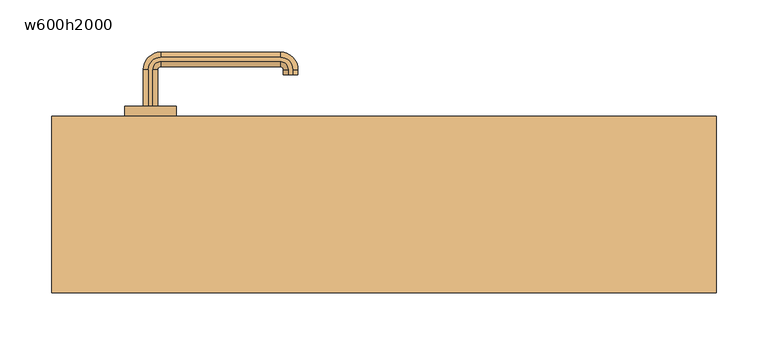
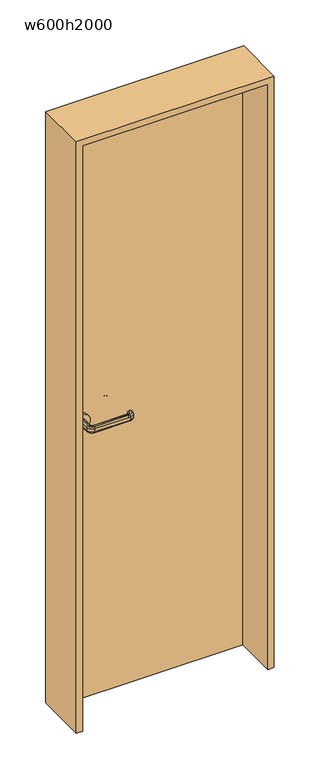
"""IFC4 building model written with IfcOpenShell, lengths in millimetres: door geometry, 片開き : w600h2000."""

from ifc_helpers import new_model, si_unit, point, frame, frame_2d, origin, origin_with_axes, place, context, project, spatial, polyline, circle_curve, ellipse_curve, trimmed, segment, composite_curve, outline, extrude, source, transform, mapped, element, save
from ifc_brep_helpers import plane_surface, cylinder_surface, revolved_surface, advanced_brep


def w600h2000_ea82102f(model_context):
    return source(origin(), model_context, "Body", "SolidModel", [
        advanced_brep(
        [(-227.0, 95.0, 960.0), (-232.0, 95.0, 955.0), (-232.0, 95.0, 945.0477623), (-227.0, 95.0, 940.0477623), (-223.0, 95.0, 940.0477623), (-218.0, 95.0, 945.0477623), (-218.0, 95.0, 955.0), (-223.0, 95.0, 960.0), (-227.0, 130.0, 960.0), (-232.0, 130.0, 955.0), (-232.0, 130.0, 945.0477623), (-227.0, 130.0, 940.0477623), (-215.0, 142.0, 940.0477623), (-100.0, 142.0, 940.0477623), (-88.0, 130.0, 940.0477623), (-88.0, 125.0, 940.0477623), (-92.0, 125.0, 940.0477623), (-92.0, 130.0, 940.0477623), (-100.0, 138.0, 940.0477623), (-215.0, 138.0, 940.0477623), (-223.0, 130.0, 940.0477623), (-218.0, 130.0, 945.0477623), (-218.0, 130.0, 955.0), (-223.0, 130.0, 960.0), (-215.0, 138.0, 960.0), (-100.0, 138.0, 960.0), (-92.0, 130.0, 960.0), (-92.0, 125.0, 960.0), (-88.0, 125.0, 960.0), (-88.0, 130.0, 960.0), (-100.0, 142.0, 960.0), (-215.0, 142.0, 960.0), (-215.0, 147.0, 955.0), (-215.0, 147.0, 945.0477623), (-215.0, 133.0, 945.0477623), (-215.0, 133.0, 955.0), (-100.0, 147.0, 955.0), (-100.0, 147.0, 945.0477623), (-100.0, 133.0, 945.0477623), (-100.0, 133.0, 955.0), (-83.0, 130.0, 955.0), (-83.0, 130.0, 945.0477623), (-97.0, 130.0, 945.0477623), (-97.0, 130.0, 955.0), (-97.0, 125.0, 955.0), (-97.0, 125.0, 945.0477623), (-83.0, 125.0, 945.0477623), (-83.0, 125.0, 955.0)],
        [
            (0, 1, circle_curve(frame((-227.0, 95.0, 955.0), z_axis=(0.0, -1.0, 0.0), x_axis=(-1.0, 0.0, 0.0)), 5.0)),
            (1, 2),
            (2, 3, circle_curve(frame((-227.0, 95.0, 945.0477623), z_axis=(0.0, -1.0, 0.0), x_axis=(-1.0, 0.0, 0.0)), 5.0)),
            (3, 4),
            (4, 5, circle_curve(frame((-223.0, 95.0, 945.0477623), z_axis=(0.0, -1.0, 0.0), x_axis=(-1.0, 0.0, 0.0)), 5.0)),
            (5, 6),
            (6, 7, circle_curve(frame((-223.0, 95.0, 955.0), z_axis=(0.0, -1.0, 0.0), x_axis=(-1.0, 0.0, 0.0)), 5.0)),
            (7, 0),
            (0, 8),
            (8, 9, circle_curve(frame((-227.0, 130.0, 955.0), z_axis=(0.0, -1.0, 0.0), x_axis=(-1.0, 0.0, 0.0)), 5.0)),
            (9, 1),
            (9, 10),
            (10, 2),
            (10, 11, circle_curve(frame((-227.0, 130.0, 945.0477623), z_axis=(0.0, -1.0, 0.0), x_axis=(-1.0, 0.0, 0.0)), 5.0)),
            (11, 3),
            (11, 12, circle_curve(frame((-215.0, 130.0, 940.0477623), z_axis=(0.0, 0.0, -1.0), x_axis=(-1.0, 0.0, 0.0)), 12.0)),
            (12, 13),
            (13, 14, circle_curve(frame((-100.0, 130.0, 940.0477623), z_axis=(0.0, 0.0, -1.0), x_axis=(0.0, 1.0, 0.0)), 12.0)),
            (14, 15),
            (15, 16),
            (16, 17),
            (17, 18, circle_curve(frame((-100.0, 130.0, 940.0477623), z_axis=(0.0, 0.0, 1.0), x_axis=(0.0, 1.0, 0.0)), 8.0)),
            (18, 19),
            (19, 20, circle_curve(frame((-215.0, 130.0, 940.0477623), z_axis=(0.0, 0.0, 1.0), x_axis=(-1.0, 0.0, 0.0)), 8.0)),
            (20, 4),
            (20, 21, circle_curve(frame((-223.0, 130.0, 945.0477623), z_axis=(0.0, -1.0, 0.0), x_axis=(-1.0, 0.0, 0.0)), 5.0)),
            (21, 5),
            (21, 22),
            (22, 6),
            (22, 23, circle_curve(frame((-223.0, 130.0, 955.0), z_axis=(0.0, -1.0, 0.0), x_axis=(-1.0, 0.0, 0.0)), 5.0)),
            (23, 7),
            (23, 24, circle_curve(frame((-215.0, 130.0, 960.0), z_axis=(0.0, 0.0, -1.0), x_axis=(-1.0, 0.0, 0.0)), 8.0)),
            (24, 25),
            (25, 26, circle_curve(frame((-100.0, 130.0, 960.0), z_axis=(0.0, 0.0, -1.0), x_axis=(0.0, 1.0, 0.0)), 8.0)),
            (26, 27),
            (27, 28),
            (28, 29),
            (29, 30, circle_curve(frame((-100.0, 130.0, 960.0), z_axis=(0.0, 0.0, 1.0), x_axis=(0.0, 1.0, 0.0)), 12.0)),
            (30, 31),
            (31, 8, circle_curve(frame((-215.0, 130.0, 960.0), z_axis=(0.0, 0.0, 1.0), x_axis=(-1.0, 0.0, 0.0)), 12.0)),
            (32, 9, circle_curve(frame((-215.0, 130.0, 955.0), z_axis=(0.0, 0.0, 1.0), x_axis=(-1.0, 0.0, 0.0)), 17.0)),
            (31, 32, circle_curve(frame((-215.0, 142.0, 955.0), z_axis=(-1.0, 0.0, 0.0), x_axis=(0.0, 1.0, 0.0)), 5.0)),
            (33, 10, circle_curve(frame((-215.0, 130.0, 945.0477623), z_axis=(0.0, 0.0, 1.0), x_axis=(-1.0, 0.0, 0.0)), 17.0)),
            (32, 33),
            (33, 12, circle_curve(frame((-215.0, 142.0, 945.0477623), z_axis=(-1.0, 0.0, 0.0), x_axis=(0.0, 1.0, 0.0)), 5.0)),
            (34, 21, circle_curve(frame((-215.0, 130.0, 945.0477623), z_axis=(0.0, 0.0, 1.0), x_axis=(-1.0, 0.0, 0.0)), 3.0)),
            (19, 34, circle_curve(frame((-215.0, 138.0, 945.0477623), z_axis=(-1.0, 0.0, 0.0), x_axis=(0.0, 1.0, 0.0)), 5.0)),
            (35, 22, circle_curve(frame((-215.0, 130.0, 955.0), z_axis=(0.0, 0.0, 1.0), x_axis=(-1.0, 0.0, 0.0)), 3.0)),
            (34, 35),
            (35, 24, circle_curve(frame((-215.0, 138.0, 955.0), z_axis=(-1.0, 0.0, 0.0), x_axis=(0.0, 1.0, 0.0)), 5.0)),
            (30, 36, circle_curve(frame((-100.0, 142.0, 955.0), z_axis=(-1.0, 0.0, 0.0), x_axis=(0.0, 1.0, 0.0)), 5.0)),
            (36, 32),
            (36, 37),
            (37, 33),
            (37, 13, circle_curve(frame((-100.0, 142.0, 945.0477623), z_axis=(-1.0, 0.0, 0.0), x_axis=(0.0, 1.0, 0.0)), 5.0)),
            (18, 38, circle_curve(frame((-100.0, 138.0, 945.0477623), z_axis=(-1.0, 0.0, 0.0), x_axis=(0.0, 1.0, 0.0)), 5.0)),
            (38, 34),
            (38, 39),
            (39, 35),
            (39, 25, circle_curve(frame((-100.0, 138.0, 955.0), z_axis=(-1.0, 0.0, 0.0), x_axis=(0.0, 1.0, 0.0)), 5.0)),
            (40, 36, circle_curve(frame((-100.0, 130.0, 955.0), z_axis=(0.0, 0.0, 1.0), x_axis=(0.0, 1.0, 0.0)), 17.0)),
            (29, 40, circle_curve(frame((-88.0, 130.0, 955.0), z_axis=(0.0, 1.0, 0.0), x_axis=(1.0, 0.0, 0.0)), 5.0)),
            (41, 37, circle_curve(frame((-100.0, 130.0, 945.0477623), z_axis=(0.0, 0.0, 1.0), x_axis=(0.0, 1.0, 0.0)), 17.0)),
            (40, 41),
            (41, 14, circle_curve(frame((-88.0, 130.0, 945.0477623), z_axis=(0.0, 1.0, 0.0), x_axis=(1.0, 0.0, 0.0)), 5.0)),
            (42, 38, circle_curve(frame((-100.0, 130.0, 945.0477623), z_axis=(0.0, 0.0, 1.0), x_axis=(0.0, 1.0, 0.0)), 3.0)),
            (17, 42, circle_curve(frame((-92.0, 130.0, 945.0477623), z_axis=(0.0, 1.0, 0.0), x_axis=(1.0, 0.0, 0.0)), 5.0)),
            (43, 39, circle_curve(frame((-100.0, 130.0, 955.0), z_axis=(0.0, 0.0, 1.0), x_axis=(0.0, 1.0, 0.0)), 3.0)),
            (42, 43),
            (43, 26, circle_curve(frame((-92.0, 130.0, 955.0), z_axis=(0.0, 1.0, 0.0), x_axis=(1.0, 0.0, 0.0)), 5.0)),
            (27, 44, circle_curve(frame((-92.0, 125.0, 955.0), z_axis=(0.0, -1.0, 0.0), x_axis=(1.0, 0.0, 0.0)), 5.0)),
            (44, 45),
            (45, 16, circle_curve(frame((-92.0, 125.0, 945.0477623), z_axis=(0.0, -1.0, 0.0), x_axis=(1.0, 0.0, 0.0)), 5.0)),
            (15, 46, circle_curve(frame((-88.0, 125.0, 945.0477623), z_axis=(0.0, -1.0, 0.0), x_axis=(1.0, 0.0, 0.0)), 5.0)),
            (46, 47),
            (47, 28, circle_curve(frame((-88.0, 125.0, 955.0), z_axis=(0.0, -1.0, 0.0), x_axis=(1.0, 0.0, 0.0)), 5.0)),
            (47, 40),
            (46, 41),
            (45, 42),
            (44, 43),
        ],
        [
            plane_surface(frame((-235.198039, 95.0, 950.0), z_axis=(0.0, -1.0, 0.0), x_axis=(0.0, 0.0, 1.0))),
            cylinder_surface(frame((-227.0, 95.0, 955.0), z_axis=(0.0, -1.0, 0.0), x_axis=(-1.0, 0.0, 0.0)), 5.0),
            plane_surface(frame((-232.0, 95.0, 955.0), z_axis=(-1.0, 0.0, 0.0), x_axis=(0.0, 1.0, 0.0))),
            cylinder_surface(frame((-227.0, 95.0, 945.0477623), z_axis=(0.0, -1.0, 0.0), x_axis=(-1.0, 0.0, 0.0)), 5.0),
            plane_surface(frame((-227.0, 95.0, 940.0477623), z_axis=(0.0, 0.0, -1.0), x_axis=(0.0, 1.0, 0.0))),
            cylinder_surface(frame((-223.0, 95.0, 945.0477623), z_axis=(0.0, -1.0, 0.0), x_axis=(-1.0, 0.0, 0.0)), 5.0),
            plane_surface(frame((-218.0, 95.0, 945.0477623), z_axis=(1.0, 0.0, 0.0), x_axis=(0.0, 1.0, 0.0))),
            cylinder_surface(frame((-223.0, 95.0, 955.0), z_axis=(0.0, -1.0, 0.0), x_axis=(-1.0, 0.0, 0.0)), 5.0),
            plane_surface(frame((-223.0, 95.0, 960.0), z_axis=(0.0, 0.0, 1.0), x_axis=(0.0, 1.0, 0.0))),
            revolved_surface(trimmed(ellipse_curve(frame((-227.0, 130.0, 955.0), z_axis=(0.0, -1.0, 0.0), x_axis=(-1.0, 0.0, 0.0)), 5.0, 5.0), [point((-227.0, 130.0, 960.0))], [point((-232.0, 130.0, 955.0))], True, "CARTESIAN"), (-215.0, 130.0, 950.0), (0.0, 0.0, -1.0)),
            cylinder_surface(frame((-215.0, 130.0, 950.0), z_axis=(0.0, 0.0, -1.0), x_axis=(-1.0, 0.0, 0.0)), 17.0),
            revolved_surface(trimmed(ellipse_curve(frame((-227.0, 130.0, 945.0477623), z_axis=(0.0, -1.0, 0.0), x_axis=(-1.0, 0.0, 0.0)), 5.0, 5.0), [point((-232.0, 130.0, 945.0477623))], [point((-227.0, 130.0, 940.0477623))], True, "CARTESIAN"), (-215.0, 130.0, 950.0), (0.0, 0.0, -1.0)),
            revolved_surface(trimmed(ellipse_curve(frame((-223.0, 130.0, 945.0477623), z_axis=(0.0, -1.0, 0.0), x_axis=(-1.0, 0.0, 0.0)), 5.0, 5.0), [point((-223.0, 130.0, 940.0477623))], [point((-218.0, 130.0, 945.0477623))], True, "CARTESIAN"), (-215.0, 130.0, 950.0), (0.0, 0.0, -1.0)),
            revolved_surface(polyline([(-218.0, 130.0, 945.0477623), (-218.0, 130.0, 955.0)]), (-215.0, 130.0, 950.0), (0.0, 0.0, -1.0)),
            revolved_surface(trimmed(ellipse_curve(frame((-223.0, 130.0, 955.0), z_axis=(0.0, -1.0, 0.0), x_axis=(-1.0, 0.0, 0.0)), 5.0, 5.0), [point((-218.0, 130.0, 955.0))], [point((-223.0, 130.0, 960.0))], True, "CARTESIAN"), (-215.0, 130.0, 950.0), (0.0, 0.0, -1.0)),
            cylinder_surface(frame((-215.0, 142.0, 955.0), z_axis=(-1.0, 0.0, 0.0), x_axis=(0.0, 1.0, 0.0)), 5.0),
            plane_surface(frame((-215.0, 147.0, 955.0), z_axis=(0.0, 1.0, 0.0), x_axis=(1.0, 0.0, 0.0))),
            cylinder_surface(frame((-215.0, 142.0, 945.0477623), z_axis=(-1.0, 0.0, 0.0), x_axis=(0.0, 1.0, 0.0)), 5.0),
            cylinder_surface(frame((-215.0, 138.0, 945.0477623), z_axis=(-1.0, 0.0, 0.0), x_axis=(0.0, 1.0, 0.0)), 5.0),
            plane_surface(frame((-215.0, 133.0, 945.0477623), z_axis=(0.0, -1.0, 0.0), x_axis=(1.0, 0.0, 0.0))),
            cylinder_surface(frame((-215.0, 138.0, 955.0), z_axis=(-1.0, 0.0, 0.0), x_axis=(0.0, 1.0, 0.0)), 5.0),
            revolved_surface(trimmed(ellipse_curve(frame((-100.0, 142.0, 955.0), z_axis=(-1.0, 0.0, 0.0), x_axis=(0.0, 1.0, 0.0)), 5.0, 5.0), [point((-100.0, 142.0, 960.0))], [point((-100.0, 147.0, 955.0))], True, "CARTESIAN"), (-100.0, 130.0, 950.0), (0.0, 0.0, -1.0)),
            cylinder_surface(frame((-100.0, 130.0, 950.0), z_axis=(0.0, 0.0, -1.0), x_axis=(0.0, 1.0, 0.0)), 17.0),
            revolved_surface(trimmed(ellipse_curve(frame((-100.0, 142.0, 945.0477623), z_axis=(-1.0, 0.0, 0.0), x_axis=(0.0, 1.0, 0.0)), 5.0, 5.0), [point((-100.0, 147.0, 945.0477623))], [point((-100.0, 142.0, 940.0477623))], True, "CARTESIAN"), (-100.0, 130.0, 950.0), (0.0, 0.0, -1.0)),
            revolved_surface(trimmed(ellipse_curve(frame((-100.0, 138.0, 945.0477623), z_axis=(-1.0, 0.0, 0.0), x_axis=(0.0, 1.0, 0.0)), 5.0, 5.0), [point((-100.0, 138.0, 940.0477623))], [point((-100.0, 133.0, 945.0477623))], True, "CARTESIAN"), (-100.0, 130.0, 950.0), (0.0, 0.0, -1.0)),
            revolved_surface(polyline([(-100.0, 133.0, 945.0477623), (-100.0, 133.0, 955.0)]), (-100.0, 130.0, 950.0), (0.0, 0.0, -1.0)),
            revolved_surface(trimmed(ellipse_curve(frame((-100.0, 138.0, 955.0), z_axis=(-1.0, 0.0, 0.0), x_axis=(0.0, 1.0, 0.0)), 5.0, 5.0), [point((-100.0, 133.0, 955.0))], [point((-100.0, 138.0, 960.0))], True, "CARTESIAN"), (-100.0, 130.0, 950.0), (0.0, 0.0, -1.0)),
            plane_surface(frame((-100.198039, 125.0, 950.0), z_axis=(0.0, -1.0, 0.0), x_axis=(0.0, 0.0, -1.0))),
            cylinder_surface(frame((-88.0, 130.0, 955.0), z_axis=(0.0, 1.0, 0.0), x_axis=(1.0, 0.0, 0.0)), 5.0),
            plane_surface(frame((-83.0, 130.0, 955.0), z_axis=(1.0, 0.0, 0.0), x_axis=(0.0, -1.0, 0.0))),
            cylinder_surface(frame((-88.0, 130.0, 945.0477623), z_axis=(0.0, 1.0, 0.0), x_axis=(1.0, 0.0, 0.0)), 5.0),
            cylinder_surface(frame((-92.0, 130.0, 945.0477623), z_axis=(0.0, 1.0, 0.0), x_axis=(1.0, 0.0, 0.0)), 5.0),
            plane_surface(frame((-97.0, 130.0, 945.0477623), z_axis=(-1.0, 0.0, 0.0), x_axis=(0.0, -1.0, 0.0))),
            cylinder_surface(frame((-92.0, 130.0, 955.0), z_axis=(0.0, 1.0, 0.0), x_axis=(1.0, 0.0, 0.0)), 5.0),
        ],
        [
            (0, [[1, 2, 3, 4, 5, 6, 7, 8]]),
            (1, [[-1, 9, 10, 11]]),
            (2, [[-2, -11, 12, 13]]),
            (3, [[-3, -13, 14, 15]]),
            (4, [[-4, -15, 16, 17, 18, 19, 20, 21, 22, 23, 24, 25]]),
            (5, [[-5, -25, 26, 27]]),
            (6, [[-6, -27, 28, 29]]),
            (7, [[-7, -29, 30, 31]]),
            (8, [[-8, -31, 32, 33, 34, 35, 36, 37, 38, 39, 40, -9]]),
            (9, [[41, -10, -40, 42]]),
            (10, [[43, -12, -41, 44]]),
            (11, [[-16, -14, -43, 45]]),
            (12, [[46, -26, -24, 47]]),
            (13, [[48, -28, -46, 49]]),
            (14, [[-32, -30, -48, 50]]),
            (15, [[-42, -39, 51, 52]]),
            (16, [[-44, -52, 53, 54]]),
            (17, [[-45, -54, 55, -17]]),
            (18, [[-47, -23, 56, 57]]),
            (19, [[-49, -57, 58, 59]]),
            (20, [[-50, -59, 60, -33]]),
            (21, [[61, -51, -38, 62]]),
            (22, [[63, -53, -61, 64]]),
            (23, [[-18, -55, -63, 65]]),
            (24, [[66, -56, -22, 67]]),
            (25, [[68, -58, -66, 69]]),
            (26, [[-34, -60, -68, 70]]),
            (27, [[-36, 71, 72, 73, -20, 74, 75, 76]]),
            (28, [[-62, -37, -76, 77]]),
            (29, [[-64, -77, -75, 78]]),
            (30, [[-65, -78, -74, -19]]),
            (31, [[-67, -21, -73, 79]]),
            (32, [[-69, -79, -72, 80]]),
            (33, [[-70, -80, -71, -35]]),
        ],
    ),
        advanced_brep(
        [(-223.0, 45.0, 940.0), (-227.0, 45.0, 940.0), (-232.0, 45.0, 945.0), (-232.0, 45.0, 955.0), (-227.0, 45.0, 960.0), (-223.0, 45.0, 960.0), (-218.0, 45.0, 955.0), (-218.0, 45.0, 945.0), (-223.0, 10.0, 940.0), (-215.0, 2.0, 940.0), (-100.0, 2.0, 940.0), (-92.0, 10.0, 940.0), (-92.0, 15.0, 940.0), (-88.0, 15.0, 940.0), (-88.0, 10.0, 940.0), (-100.0, -2.0, 940.0), (-215.0, -2.0, 940.0), (-227.0, 10.0, 940.0), (-232.0, 10.0, 945.0), (-232.0, 10.0, 955.0), (-227.0, 10.0, 960.0), (-215.0, -2.0, 960.0), (-100.0, -2.0, 960.0), (-88.0, 10.0, 960.0), (-88.0, 15.0, 960.0), (-92.0, 15.0, 960.0), (-92.0, 10.0, 960.0), (-100.0, 2.0, 960.0), (-215.0, 2.0, 960.0), (-223.0, 10.0, 960.0), (-218.0, 10.0, 955.0), (-218.0, 10.0, 945.0), (-215.0, -7.0, 945.0), (-215.0, -7.0, 955.0), (-215.0, 7.0, 955.0), (-215.0, 7.0, 945.0), (-100.0, -7.0, 945.0), (-100.0, -7.0, 955.0), (-100.0, 7.0, 955.0), (-100.0, 7.0, 945.0), (-83.0, 10.0, 945.0), (-83.0, 10.0, 955.0), (-97.0, 10.0, 955.0), (-97.0, 10.0, 945.0), (-97.0, 15.0, 945.0), (-97.0, 15.0, 955.0), (-83.0, 15.0, 955.0), (-83.0, 15.0, 945.0)],
        [
            (0, 1),
            (1, 2, circle_curve(frame((-227.0, 45.0, 945.0), z_axis=(0.0, 1.0, 0.0), x_axis=(1.0, 0.0, 0.0)), 5.0)),
            (2, 3),
            (3, 4, circle_curve(frame((-227.0, 45.0, 955.0), z_axis=(0.0, 1.0, 0.0), x_axis=(1.0, 0.0, 0.0)), 5.0)),
            (4, 5),
            (5, 6, circle_curve(frame((-223.0, 45.0, 955.0), z_axis=(0.0, 1.0, 0.0), x_axis=(1.0, 0.0, 0.0)), 5.0)),
            (6, 7),
            (7, 0, circle_curve(frame((-223.0, 45.0, 945.0), z_axis=(0.0, 1.0, 0.0), x_axis=(1.0, 0.0, 0.0)), 5.0)),
            (0, 8),
            (8, 9, circle_curve(frame((-215.0, 10.0, 940.0), z_axis=(0.0, 0.0, 1.0), x_axis=(-1.0, 0.0, 0.0)), 8.0)),
            (9, 10),
            (10, 11, circle_curve(frame((-100.0, 10.0, 940.0), z_axis=(0.0, 0.0, 1.0), x_axis=(0.0, -1.0, 0.0)), 8.0)),
            (11, 12),
            (12, 13),
            (13, 14),
            (14, 15, circle_curve(frame((-100.0, 10.0, 940.0), z_axis=(0.0, 0.0, -1.0), x_axis=(0.0, -1.0, 0.0)), 12.0)),
            (15, 16),
            (16, 17, circle_curve(frame((-215.0, 10.0, 940.0), z_axis=(0.0, 0.0, -1.0), x_axis=(-1.0, 0.0, 0.0)), 12.0)),
            (17, 1),
            (17, 18, circle_curve(frame((-227.0, 10.0, 945.0), z_axis=(0.0, 1.0, 0.0), x_axis=(1.0, 0.0, 0.0)), 5.0)),
            (18, 2),
            (18, 19),
            (19, 3),
            (19, 20, circle_curve(frame((-227.0, 10.0, 955.0), z_axis=(0.0, 1.0, 0.0), x_axis=(1.0, 0.0, 0.0)), 5.0)),
            (20, 4),
            (20, 21, circle_curve(frame((-215.0, 10.0, 960.0), z_axis=(0.0, 0.0, 1.0), x_axis=(-1.0, 0.0, 0.0)), 12.0)),
            (21, 22),
            (22, 23, circle_curve(frame((-100.0, 10.0, 960.0), z_axis=(0.0, 0.0, 1.0), x_axis=(0.0, -1.0, 0.0)), 12.0)),
            (23, 24),
            (24, 25),
            (25, 26),
            (26, 27, circle_curve(frame((-100.0, 10.0, 960.0), z_axis=(0.0, 0.0, -1.0), x_axis=(0.0, -1.0, 0.0)), 8.0)),
            (27, 28),
            (28, 29, circle_curve(frame((-215.0, 10.0, 960.0), z_axis=(0.0, 0.0, -1.0), x_axis=(-1.0, 0.0, 0.0)), 8.0)),
            (29, 5),
            (29, 30, circle_curve(frame((-223.0, 10.0, 955.0), z_axis=(0.0, 1.0, 0.0), x_axis=(1.0, 0.0, 0.0)), 5.0)),
            (30, 6),
            (30, 31),
            (31, 7),
            (31, 8, circle_curve(frame((-223.0, 10.0, 945.0), z_axis=(0.0, 1.0, 0.0), x_axis=(1.0, 0.0, 0.0)), 5.0)),
            (32, 18, circle_curve(frame((-215.0, 10.0, 945.0), z_axis=(0.0, 0.0, -1.0), x_axis=(-1.0, 0.0, 0.0)), 17.0)),
            (16, 32, circle_curve(frame((-215.0, -2.0, 945.0), z_axis=(-1.0, 0.0, 0.0), x_axis=(0.0, 1.0, 0.0)), 5.0)),
            (33, 19, circle_curve(frame((-215.0, 10.0, 955.0), z_axis=(0.0, 0.0, -1.0), x_axis=(-1.0, 0.0, 0.0)), 17.0)),
            (32, 33),
            (33, 21, circle_curve(frame((-215.0, -2.0, 955.0), z_axis=(-1.0, 0.0, 0.0), x_axis=(0.0, 1.0, 0.0)), 5.0)),
            (34, 30, circle_curve(frame((-215.0, 10.0, 955.0), z_axis=(0.0, 0.0, -1.0), x_axis=(-1.0, 0.0, 0.0)), 3.0)),
            (28, 34, circle_curve(frame((-215.0, 2.0, 955.0), z_axis=(-1.0, 0.0, 0.0), x_axis=(0.0, 1.0, 0.0)), 5.0)),
            (35, 31, circle_curve(frame((-215.0, 10.0, 945.0), z_axis=(0.0, 0.0, -1.0), x_axis=(-1.0, 0.0, 0.0)), 3.0)),
            (34, 35),
            (35, 9, circle_curve(frame((-215.0, 2.0, 945.0), z_axis=(-1.0, 0.0, 0.0), x_axis=(0.0, 1.0, 0.0)), 5.0)),
            (15, 36, circle_curve(frame((-100.0, -2.0, 945.0), z_axis=(-1.0, 0.0, 0.0), x_axis=(0.0, 1.0, 0.0)), 5.0)),
            (36, 32),
            (36, 37),
            (37, 33),
            (37, 22, circle_curve(frame((-100.0, -2.0, 955.0), z_axis=(-1.0, 0.0, 0.0), x_axis=(0.0, 1.0, 0.0)), 5.0)),
            (27, 38, circle_curve(frame((-100.0, 2.0, 955.0), z_axis=(-1.0, 0.0, 0.0), x_axis=(0.0, 1.0, 0.0)), 5.0)),
            (38, 34),
            (38, 39),
            (39, 35),
            (39, 10, circle_curve(frame((-100.0, 2.0, 945.0), z_axis=(-1.0, 0.0, 0.0), x_axis=(0.0, 1.0, 0.0)), 5.0)),
            (40, 36, circle_curve(frame((-100.0, 10.0, 945.0), z_axis=(0.0, 0.0, -1.0), x_axis=(0.0, -1.0, 0.0)), 17.0)),
            (14, 40, circle_curve(frame((-88.0, 10.0, 945.0), z_axis=(0.0, -1.0, 0.0), x_axis=(-1.0, 0.0, 0.0)), 5.0)),
            (41, 37, circle_curve(frame((-100.0, 10.0, 955.0), z_axis=(0.0, 0.0, -1.0), x_axis=(0.0, -1.0, 0.0)), 17.0)),
            (40, 41),
            (41, 23, circle_curve(frame((-88.0, 10.0, 955.0), z_axis=(0.0, -1.0, 0.0), x_axis=(-1.0, 0.0, 0.0)), 5.0)),
            (42, 38, circle_curve(frame((-100.0, 10.0, 955.0), z_axis=(0.0, 0.0, -1.0), x_axis=(0.0, -1.0, 0.0)), 3.0)),
            (26, 42, circle_curve(frame((-92.0, 10.0, 955.0), z_axis=(0.0, -1.0, 0.0), x_axis=(-1.0, 0.0, 0.0)), 5.0)),
            (43, 39, circle_curve(frame((-100.0, 10.0, 945.0), z_axis=(0.0, 0.0, -1.0), x_axis=(0.0, -1.0, 0.0)), 3.0)),
            (42, 43),
            (43, 11, circle_curve(frame((-92.0, 10.0, 945.0), z_axis=(0.0, -1.0, 0.0), x_axis=(-1.0, 0.0, 0.0)), 5.0)),
            (12, 44, circle_curve(frame((-92.0, 15.0, 945.0), z_axis=(0.0, 1.0, 0.0), x_axis=(-1.0, 0.0, 0.0)), 5.0)),
            (44, 45),
            (45, 25, circle_curve(frame((-92.0, 15.0, 955.0), z_axis=(0.0, 1.0, 0.0), x_axis=(-1.0, 0.0, 0.0)), 5.0)),
            (24, 46, circle_curve(frame((-88.0, 15.0, 955.0), z_axis=(0.0, 1.0, 0.0), x_axis=(-1.0, 0.0, 0.0)), 5.0)),
            (46, 47),
            (47, 13, circle_curve(frame((-88.0, 15.0, 945.0), z_axis=(0.0, 1.0, 0.0), x_axis=(-1.0, 0.0, 0.0)), 5.0)),
            (47, 40),
            (46, 41),
            (45, 42),
            (44, 43),
        ],
        [
            plane_surface(frame((-235.198039, 45.0, 950.0), z_axis=(0.0, 1.0, 0.0), x_axis=(0.0, 0.0, -1.0))),
            plane_surface(frame((-223.0, 45.0, 940.0), z_axis=(0.0, 0.0, -1.0), x_axis=(0.0, -1.0, 0.0))),
            cylinder_surface(frame((-227.0, 45.0, 945.0), z_axis=(0.0, 1.0, 0.0), x_axis=(1.0, 0.0, 0.0)), 5.0),
            plane_surface(frame((-232.0, 45.0, 945.0), z_axis=(-1.0, 0.0, 0.0), x_axis=(0.0, -1.0, 0.0))),
            cylinder_surface(frame((-227.0, 45.0, 955.0), z_axis=(0.0, 1.0, 0.0), x_axis=(1.0, 0.0, 0.0)), 5.0),
            plane_surface(frame((-227.0, 45.0, 960.0), z_axis=(0.0, 0.0, 1.0), x_axis=(0.0, -1.0, 0.0))),
            cylinder_surface(frame((-223.0, 45.0, 955.0), z_axis=(0.0, 1.0, 0.0), x_axis=(1.0, 0.0, 0.0)), 5.0),
            plane_surface(frame((-218.0, 45.0, 955.0), z_axis=(1.0, 0.0, 0.0), x_axis=(0.0, -1.0, 0.0))),
            cylinder_surface(frame((-223.0, 45.0, 945.0), z_axis=(0.0, 1.0, 0.0), x_axis=(1.0, 0.0, 0.0)), 5.0),
            revolved_surface(trimmed(ellipse_curve(frame((-227.0, 10.0, 945.0), z_axis=(0.0, 1.0, 0.0), x_axis=(1.0, 0.0, 0.0)), 5.0, 5.0), [point((-227.0, 10.0, 940.0))], [point((-232.0, 10.0, 945.0))], True, "CARTESIAN"), (-215.0, 10.0, 950.0), (0.0, 0.0, 1.0)),
            cylinder_surface(frame((-215.0, 10.0, 950.0), z_axis=(0.0, 0.0, 1.0), x_axis=(-1.0, 0.0, 0.0)), 17.0),
            revolved_surface(trimmed(ellipse_curve(frame((-227.0, 10.0, 955.0), z_axis=(0.0, 1.0, 0.0), x_axis=(1.0, 0.0, 0.0)), 5.0, 5.0), [point((-232.0, 10.0, 955.0))], [point((-227.0, 10.0, 960.0))], True, "CARTESIAN"), (-215.0, 10.0, 950.0), (0.0, 0.0, 1.0)),
            revolved_surface(trimmed(ellipse_curve(frame((-223.0, 10.0, 955.0), z_axis=(0.0, 1.0, 0.0), x_axis=(1.0, 0.0, 0.0)), 5.0, 5.0), [point((-223.0, 10.0, 960.0))], [point((-218.0, 10.0, 955.0))], True, "CARTESIAN"), (-215.0, 10.0, 950.0), (0.0, 0.0, 1.0)),
            revolved_surface(polyline([(-218.0, 10.0, 955.0), (-218.0, 10.0, 945.0)]), (-215.0, 10.0, 950.0), (0.0, 0.0, 1.0)),
            revolved_surface(trimmed(ellipse_curve(frame((-223.0, 10.0, 945.0), z_axis=(0.0, 1.0, 0.0), x_axis=(1.0, 0.0, 0.0)), 5.0, 5.0), [point((-218.0, 10.0, 945.0))], [point((-223.0, 10.0, 940.0))], True, "CARTESIAN"), (-215.0, 10.0, 950.0), (0.0, 0.0, 1.0)),
            cylinder_surface(frame((-215.0, -2.0, 945.0), z_axis=(-1.0, 0.0, 0.0), x_axis=(0.0, 1.0, 0.0)), 5.0),
            plane_surface(frame((-215.0, -7.0, 945.0), z_axis=(0.0, -1.0, 0.0), x_axis=(1.0, 0.0, 0.0))),
            cylinder_surface(frame((-215.0, -2.0, 955.0), z_axis=(-1.0, 0.0, 0.0), x_axis=(0.0, 1.0, 0.0)), 5.0),
            cylinder_surface(frame((-215.0, 2.0, 955.0), z_axis=(-1.0, 0.0, 0.0), x_axis=(0.0, 1.0, 0.0)), 5.0),
            plane_surface(frame((-215.0, 7.0, 955.0), z_axis=(0.0, 1.0, 0.0), x_axis=(1.0, 0.0, 0.0))),
            cylinder_surface(frame((-215.0, 2.0, 945.0), z_axis=(-1.0, 0.0, 0.0), x_axis=(0.0, 1.0, 0.0)), 5.0),
            revolved_surface(trimmed(ellipse_curve(frame((-100.0, -2.0, 945.0), z_axis=(-1.0, 0.0, 0.0), x_axis=(0.0, 1.0, 0.0)), 5.0, 5.0), [point((-100.0, -2.0, 940.0))], [point((-100.0, -7.0, 945.0))], True, "CARTESIAN"), (-100.0, 10.0, 950.0), (0.0, 0.0, 1.0)),
            cylinder_surface(frame((-100.0, 10.0, 950.0), z_axis=(0.0, 0.0, 1.0), x_axis=(0.0, -1.0, 0.0)), 17.0),
            revolved_surface(trimmed(ellipse_curve(frame((-100.0, -2.0, 955.0), z_axis=(-1.0, 0.0, 0.0), x_axis=(0.0, 1.0, 0.0)), 5.0, 5.0), [point((-100.0, -7.0, 955.0))], [point((-100.0, -2.0, 960.0))], True, "CARTESIAN"), (-100.0, 10.0, 950.0), (0.0, 0.0, 1.0)),
            revolved_surface(trimmed(ellipse_curve(frame((-100.0, 2.0, 955.0), z_axis=(-1.0, 0.0, 0.0), x_axis=(0.0, 1.0, 0.0)), 5.0, 5.0), [point((-100.0, 2.0, 960.0))], [point((-100.0, 7.0, 955.0))], True, "CARTESIAN"), (-100.0, 10.0, 950.0), (0.0, 0.0, 1.0)),
            revolved_surface(polyline([(-100.0, 7.0, 955.0), (-100.0, 7.0, 945.0)]), (-100.0, 10.0, 950.0), (0.0, 0.0, 1.0)),
            revolved_surface(trimmed(ellipse_curve(frame((-100.0, 2.0, 945.0), z_axis=(-1.0, 0.0, 0.0), x_axis=(0.0, 1.0, 0.0)), 5.0, 5.0), [point((-100.0, 7.0, 945.0))], [point((-100.0, 2.0, 940.0))], True, "CARTESIAN"), (-100.0, 10.0, 950.0), (0.0, 0.0, 1.0)),
            plane_surface(frame((-100.198039, 15.0, 950.0), z_axis=(0.0, 1.0, 0.0), x_axis=(0.0, 0.0, 1.0))),
            cylinder_surface(frame((-88.0, 10.0, 945.0), z_axis=(0.0, -1.0, 0.0), x_axis=(-1.0, 0.0, 0.0)), 5.0),
            plane_surface(frame((-83.0, 10.0, 945.0), z_axis=(1.0, 0.0, 0.0), x_axis=(0.0, 1.0, 0.0))),
            cylinder_surface(frame((-88.0, 10.0, 955.0), z_axis=(0.0, -1.0, 0.0), x_axis=(-1.0, 0.0, 0.0)), 5.0),
            cylinder_surface(frame((-92.0, 10.0, 955.0), z_axis=(0.0, -1.0, 0.0), x_axis=(-1.0, 0.0, 0.0)), 5.0),
            plane_surface(frame((-97.0, 10.0, 955.0), z_axis=(-1.0, 0.0, 0.0), x_axis=(0.0, 1.0, 0.0))),
            cylinder_surface(frame((-92.0, 10.0, 945.0), z_axis=(0.0, -1.0, 0.0), x_axis=(-1.0, 0.0, 0.0)), 5.0),
        ],
        [
            (0, [[1, 2, 3, 4, 5, 6, 7, 8]]),
            (1, [[-1, 9, 10, 11, 12, 13, 14, 15, 16, 17, 18, 19]]),
            (2, [[-2, -19, 20, 21]]),
            (3, [[-3, -21, 22, 23]]),
            (4, [[-4, -23, 24, 25]]),
            (5, [[-5, -25, 26, 27, 28, 29, 30, 31, 32, 33, 34, 35]]),
            (6, [[-6, -35, 36, 37]]),
            (7, [[-7, -37, 38, 39]]),
            (8, [[-8, -39, 40, -9]]),
            (9, [[41, -20, -18, 42]]),
            (10, [[43, -22, -41, 44]]),
            (11, [[-26, -24, -43, 45]]),
            (12, [[46, -36, -34, 47]]),
            (13, [[48, -38, -46, 49]]),
            (14, [[-10, -40, -48, 50]]),
            (15, [[-42, -17, 51, 52]]),
            (16, [[-44, -52, 53, 54]]),
            (17, [[-45, -54, 55, -27]]),
            (18, [[-47, -33, 56, 57]]),
            (19, [[-49, -57, 58, 59]]),
            (20, [[-50, -59, 60, -11]]),
            (21, [[61, -51, -16, 62]]),
            (22, [[63, -53, -61, 64]]),
            (23, [[-28, -55, -63, 65]]),
            (24, [[66, -56, -32, 67]]),
            (25, [[68, -58, -66, 69]]),
            (26, [[-12, -60, -68, 70]]),
            (27, [[71, 72, 73, -30, 74, 75, 76, -14]]),
            (28, [[-62, -15, -76, 77]]),
            (29, [[-64, -77, -75, 78]]),
            (30, [[-65, -78, -74, -29]]),
            (31, [[-67, -31, -73, 79]]),
            (32, [[-69, -79, -72, 80]]),
            (33, [[-70, -80, -71, -13]]),
        ],
    ),
        extrude(outline(composite_curve([segment(trimmed(circle_curve(frame_2d((950.0, -225.0)), 25.0), [point((950.0, -250.0))], [point((950.0, -200.0))], False, "CARTESIAN"), True, "CONTINUOUS"), segment(trimmed(circle_curve(frame_2d((950.0, -225.0)), 25.0), [point((950.0, -200.0))], [point((950.0, -250.0))], False, "CARTESIAN"), True, "CONTINUOUS")], self_intersect=False)), frame((0.0, 85.0, 0.0), z_axis=(0.0, 1.0, 0.0), x_axis=(0.0, 0.0, 1.0)), (0.0, 0.0, 1.0), 10.0),
        extrude(outline(composite_curve([segment(trimmed(circle_curve(frame_2d((950.0, -225.0)), 25.0), [point((950.0, -250.0))], [point((950.0, -200.0))], False, "CARTESIAN"), True, "CONTINUOUS"), segment(trimmed(circle_curve(frame_2d((950.0, -225.0)), 25.0), [point((950.0, -200.0))], [point((950.0, -250.0))], False, "CARTESIAN"), True, "CONTINUOUS")], self_intersect=False)), frame((0.0, 45.0, 0.0), z_axis=(0.0, 1.0, 0.0), x_axis=(0.0, 0.0, 1.0)), (0.0, 0.0, 1.0), 10.0),
        extrude(outline(polyline([(2020.0, -320.0), (0.0, -320.0), (0.0, -300.0), (2000.0, -300.0), (2000.0, 300.0), (0.0, 300.0), (0.0, 320.0), (2020.0, 320.0), (2020.0, -320.0)])), frame((0.0, -85.0, 0.0), z_axis=(0.0, 1.0, 0.0), x_axis=(0.0, 0.0, 1.0)), (0.0, 0.0, 1.0), 170.0),
        extrude(outline(polyline([(300.0, 55.0), (-300.0, 55.0), (-300.0, 85.0), (300.0, 85.0), (300.0, 55.0)])), origin_with_axes(), (0.0, 0.0, 1.0), 2000.0),
    ])


if __name__ == "__main__":
    model = new_model("IFC4")
    model_context = context("Model", 3, world=origin())
    ifc_project = project(units=[si_unit("LENGTHUNIT", "METRE", prefix="MILLI")], contexts=[model_context])
    site = spatial("IfcSite", under=ifc_project)
    building = spatial("IfcBuilding", under=site)
    placement = place(None, origin())
    w600h2000_shape = w600h2000_ea82102f(model_context)
    element("IfcDoor", 1, ObjectType="片開き : w600h2000", at=placement, inside=building, context=model_context, shape_type="MappedRepresentation", body=[
        mapped(w600h2000_shape, transform((0.0, 0.0, 0.0), x_axis=(1.0, 0.0, 0.0), y_axis=(0.0, 1.0, 0.0), z_axis=(0.0, 0.0, 1.0))),
    ])
    save(model, "model.ifc")

# Revit data of these elements
# Type "片開き : w600h2000"
#   Construction Type Id = "MDOOR"
#   Analytic Construction = "メタル"
#   Type Mark = "49"
#   Operation = "片側開き戸右"
#   Keynote = "08110.P2"
#   Visual Light Transmittance = 0
#   Solar Heat Gain Coefficient = 0
#   Heat Transfer Coefficient (U) = 3.7021 W/(m²·K)
#   高さ(中心) = 1000 mm
#   Height = 2000 mm
#   Thickness = 30 mm
#   ドア枠見附 = 20 mm
#   Width = 600 mm
#   取手取付け高さ = 950 mm
#   ドア枠ちり = 10 mm
#   Function = 0
#   ドア枠 [instance default] = 塗装ホワイト
#   ドア把手 [instance default] = メタル-ステンレス
#   ドア [instance default] = 塗装ホワイト
#   Wall Closure = (empty or 0)
# Element 1 (IfcDoor, "片開き : w600h2000")
#   Materials on its faces: "メタル-ステンレス", "塗装ホワイト"
# Materials
#   "塗装ホワイト": class "ペイント", colour RGB 249 249 249, transparency 0, Cost = 0
#   "メタル-ステンレス": class "メタル", colour RGB 247 247 247, transparency 0, Cost = 0
